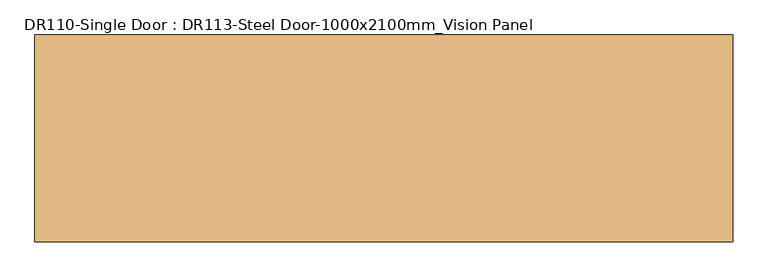
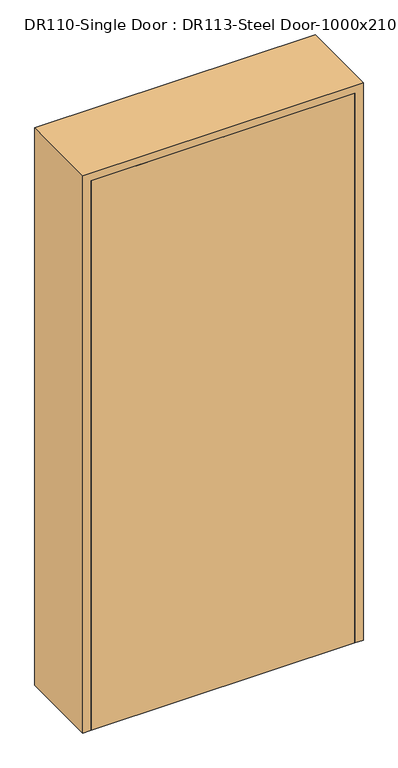
"""IFC4 building model written with IfcOpenShell, lengths in millimetres: door geometry, DR110-Single Door : DR113-Steel Door-1000x2100mm_Vision Panel."""

from ifc_helpers import new_model, si_unit, origin, origin_with_axes, place, context, project, spatial, polyline, outline, extrude, faceted_brep, source, transform, mapped, element, save


def dr110_single_door_dr113_steel_door_1000x2100mm_vision_panel_7d846780(model_context):
    return source(origin(), model_context, "Body", "SolidModel", [
        extrude(outline(polyline([(470.0, -148.0), (-470.0, -148.0), (-470.0, -113.0), (470.0, -113.0), (470.0, -148.0)])), origin_with_axes(), (0.0, 0.0, 1.0), 2070.0),
        faceted_brep([(470.0, -148.0, 0.0), (470.0, -113.0, 0.0), (450.0, -113.0, 0.0), (450.0, 113.0, 0.0), (470.0, 113.0, 0.0), (470.0, 148.0, 0.0), (500.0, 148.0, 0.0), (500.0, -148.0, 0.0), (500.0, -148.0, 2100.0), (-500.0, -148.0, 2100.0), (-500.0, -148.0, 0.0), (-470.0, -148.0, 0.0), (-470.0, -148.0, 2070.0), (470.0, -148.0, 2070.0), (500.0, 148.0, 2100.0), (470.0, 148.0, 2070.0), (-470.0, 148.0, 2070.0), (-470.0, 148.0, 0.0), (-500.0, 148.0, 0.0), (-500.0, 148.0, 2100.0), (470.0, 113.0, 2070.0), (450.0, 113.0, 2050.0), (-450.0, 113.0, 2050.0), (-450.0, 113.0, 0.0), (-470.0, 113.0, 0.0), (-470.0, 113.0, 2070.0), (450.0, -113.0, 2050.0), (470.0, -113.0, 2070.0), (-470.0, -113.0, 2070.0), (-470.0, -113.0, 0.0), (-450.0, -113.0, 0.0), (-450.0, -113.0, 2050.0)], [[[0, 1, 2, 3, 4, 5, 6, 7]], [[7, 8, 9, 10, 11, 12, 13, 0]], [[6, 14, 8, 7]], [[5, 15, 16, 17, 18, 19, 14, 6]], [[4, 20, 15, 5]], [[3, 21, 22, 23, 24, 25, 20, 4]], [[2, 26, 21, 3]], [[1, 27, 28, 29, 30, 31, 26, 2]], [[0, 13, 27, 1]], [[12, 11, 29, 28]], [[11, 10, 18, 17, 24, 23, 30, 29]], [[19, 18, 10, 9]], [[25, 24, 17, 16]], [[31, 30, 23, 22]], [[14, 19, 9, 8]], [[20, 25, 16, 15]], [[26, 31, 22, 21]], [[13, 12, 28, 27]]]),
    ])


if __name__ == "__main__":
    model = new_model("IFC4")
    model_context = context("Model", 3, world=origin())
    ifc_project = project(units=[si_unit("LENGTHUNIT", "METRE", prefix="MILLI")], contexts=[model_context])
    site = spatial("IfcSite", under=ifc_project)
    building = spatial("IfcBuilding", under=site)
    placement = place(None, origin())
    dr110_single_door_dr113_steel_door_1000x2100mm_vision_panel_shape = dr110_single_door_dr113_steel_door_1000x2100mm_vision_panel_7d846780(model_context)
    element("IfcDoor", 1, ObjectType="DR110-Single Door : DR113-Steel Door-1000x2100mm_Vision Panel", at=placement, inside=building, context=model_context, shape_type="MappedRepresentation", body=[
        mapped(dr110_single_door_dr113_steel_door_1000x2100mm_vision_panel_shape, transform((0.0, 0.0, 0.0), x_axis=(1.0, 0.0, 0.0), y_axis=(0.0, 1.0, 0.0), z_axis=(0.0, 0.0, 1.0))),
    ])
    save(model, "model.ifc")

# Revit data of these elements
# Type "DR110-Single Door : DR113-Steel Door-1000x2100mm_Vision Panel"
#   Type Mark = "SD"
#   Analytic Construction = "<None>"
#   프레임 투영 외부. = 25 mm
#   프레임 투영 내부. = 25 mm
#   프레임 폭 = 75 mm
#   Height = 2100 mm
#   Width = 1000 mm
#   Define Thermal Properties by = 1
#   문 패널 = SD1 문 패널
#   문 프레임 = A04AQ098-00002_Steel Door_non FP_single
#   Function = (empty or 0)
#   Wall Closure = (empty or 0)
# Element 1 (IfcDoor, "DR110-Single Door : DR113-Steel Door-1000x2100mm_Vision Panel")
#   Materials on its faces: "A04AQ098-00002_Steel Door_non FP_single", "SD1 문 패널"
# Materials
#   "SD1 문 패널": class "금속", colour RGB 247 247 247, transparency 0, Description = "STEEL DOOR (1000Wx2100H)"
#   "A04AQ098-00002_Steel Door_non FP_single": class "금속", colour RGB 247 247 247, transparency 0, Description = "Steel Door", W00) Work Master Code = "A04AQ098-00002", W01) Work Master_Lv1 = "Finishing Work", W02) Work Master_Lv2 = "Door & Window Work", W03) Work Master_Spec.1 = "Steel Door w/ Steel Frame", W04) Work Master_Spec.2 = "Fire Protective Rating: N/A, Single Door", W05) Work Master_Spec.3 = "w/ Hardware & Accessories", Cost = 0
